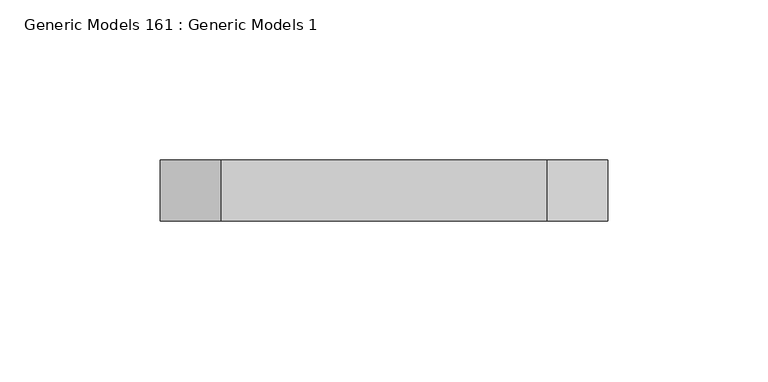
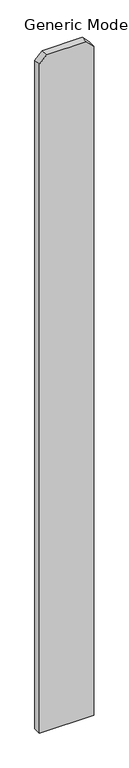
"""IFC4 building model written with IfcOpenShell, lengths in millimetres: proxy geometry, Generic Models 161 : Generic Models 1."""

import ifcopenshell
import ifcopenshell.guid

model = None  # the IFC model being written
_history = None  # IfcOwnerHistory: only IFC2X3 demands one
_inside = {}  # id of a spatial element -> (the spatial element, [elements in it])
_under = {}  # id of a project, library or spatial element -> (it, [spatial elements below it])
_declared = {}  # id of a project -> (the project, [libraries it declares])
_typed = {}  # id of a type object -> (the type object, [elements of that type])
_made_of = {}  # id of a material, layer set ... -> (it, [elements and type objects made of it])


def new_model(schema):
    """Start an empty IFC model of exactly this schema.

    Asked for "IFC4X3", IfcOpenShell would pick the latest addendum, in which some entities
    have other attributes; the version numbers below select the first issue.
    IFC2X3 requires an IfcOwnerHistory on every rooted entity: one is made here for all.
    """
    global model, _history
    if schema == "IFC4X3":
        model = ifcopenshell.file(schema_version=(4, 3, 0, 0))
    else:
        model = ifcopenshell.file(schema=schema)
    _inside.clear()
    _under.clear()
    _declared.clear()
    _typed.clear()
    _made_of.clear()
    _history = None
    if model.schema == "IFC2X3":
        org = make("IfcOrganization", Name="unknown")
        user = make(
            "IfcPersonAndOrganization",
            ThePerson=make("IfcPerson", FamilyName="unknown"),
            TheOrganization=org,
        )
        app = make(
            "IfcApplication",
            ApplicationDeveloper=org,
            Version="unknown",
            ApplicationFullName="unknown",
            ApplicationIdentifier="unknown",
        )
        _history = make(
            "IfcOwnerHistory",
            OwningUser=user,
            OwningApplication=app,
            ChangeAction="ADDED",
            CreationDate=0,
        )
    return model


def make(cls, **values):
    """One entity of the class cls with the attributes given. An attribute that is None is left unset."""
    return model.create_entity(
        cls, **{name: value for name, value in values.items() if value is not None}
    )


def rooted(cls, **values):
    """An entity with a GlobalId (a new one), such as an element, a storey or a relation."""
    return make(cls, GlobalId=ifcopenshell.guid.new(), OwnerHistory=_history, **values)


def si_unit(unit_type, name, prefix=None):
    """IfcSIUnit, for example si_unit("LENGTHUNIT", "METRE", prefix="MILLI")."""
    return make("IfcSIUnit", UnitType=unit_type, Prefix=prefix, Name=name)


def assignment(units):
    """IfcUnitAssignment: the units of a project."""
    return None if units is None else make("IfcUnitAssignment", Units=units)


def point(xyz):
    """IfcCartesianPoint."""
    return None if xyz is None else make("IfcCartesianPoint", Coordinates=xyz)


def direction(xyz):
    """IfcDirection."""
    return None if xyz is None else make("IfcDirection", DirectionRatios=xyz)


def frame(location, z_axis=None, x_axis=None):
    """IfcAxis2Placement3D, a coordinate frame: its origin and axes. An axis left out is left unset."""
    return make(
        "IfcAxis2Placement3D",
        Location=point(location),
        Axis=direction(z_axis),
        RefDirection=direction(x_axis),
    )


def origin():
    """The frame at (0, 0, 0) with its axes left unset."""
    return frame((0.0, 0.0, 0.0))


def place(relative_to, where):
    """IfcLocalPlacement: puts the frame where relative to a parent placement (None: the world)."""
    return make(
        "IfcLocalPlacement", PlacementRelTo=relative_to, RelativePlacement=where
    )


def context(
    kind, dimensions, precision=None, world=None, true_north=None, identifier=None
):
    """IfcGeometricRepresentationContext, for example the 3D "Model" context."""
    return make(
        "IfcGeometricRepresentationContext",
        ContextIdentifier=identifier,
        ContextType=kind,
        CoordinateSpaceDimension=dimensions,
        Precision=precision,
        WorldCoordinateSystem=world,
        TrueNorth=true_north,
    )


def project(units=None, contexts=None):
    """IfcProject with its units and contexts."""
    return rooted(
        "IfcProject",
        Name="project",
        RepresentationContexts=contexts,
        UnitsInContext=assignment(units),
    )


def spatial(cls, under=None, at=None, **own):
    """A site, building, storey or space (cls), placed at a placement, below another one or the project."""
    s = rooted(cls, ObjectPlacement=at, **own)
    if under is not None:
        _under.setdefault(under.id(), (under, []))[1].append(s)
    return s


def polyline(points):
    """IfcPolyline through the points."""
    return make("IfcPolyline", Points=[point(p) for p in points])


def outline(outer, holes=None, kind="AREA"):
    """IfcArbitraryClosedProfileDef: a profile drawn as a closed curve; with holes, ...WithVoids."""
    if holes is None:
        return make("IfcArbitraryClosedProfileDef", ProfileType=kind, OuterCurve=outer)
    return make(
        "IfcArbitraryProfileDefWithVoids",
        ProfileType=kind,
        OuterCurve=outer,
        InnerCurves=holes,
    )


def extrude(swept, where, along, depth):
    """IfcExtrudedAreaSolid: the profile swept, set in the frame where, extruded along a direction by depth."""
    return make(
        "IfcExtrudedAreaSolid",
        SweptArea=swept,
        Position=where,
        ExtrudedDirection=direction(along),
        Depth=depth,
    )


def shape(context_of_items, identifier, shape_type, items):
    """IfcShapeRepresentation: the items that make up one representation, for example the "Body"."""
    return make(
        "IfcShapeRepresentation",
        ContextOfItems=context_of_items,
        RepresentationIdentifier=identifier,
        RepresentationType=shape_type,
        Items=items,
    )


def source(mapping_origin, context_of_items, identifier, shape_type, items):
    """IfcRepresentationMap: a shape defined once, which mapped items show again and again."""
    return make(
        "IfcRepresentationMap",
        MappingOrigin=mapping_origin,
        MappedRepresentation=shape(context_of_items, identifier, shape_type, items),
    )


def transform(
    local_origin,
    x_axis=None,
    y_axis=None,
    z_axis=None,
    scale=None,
    scale2=None,
    scale3=None,
    uniform=True,
):
    """IfcCartesianTransformationOperator3D, or its non-uniform kind. x_axis, y_axis, z_axis: its Axis1, 2, 3."""
    if uniform:
        return make(
            "IfcCartesianTransformationOperator3D",
            Axis1=direction(x_axis),
            Axis2=direction(y_axis),
            LocalOrigin=point(local_origin),
            Scale=scale,
            Axis3=direction(z_axis),
        )
    return make(
        "IfcCartesianTransformationOperator3DnonUniform",
        Axis1=direction(x_axis),
        Axis2=direction(y_axis),
        LocalOrigin=point(local_origin),
        Scale=scale,
        Axis3=direction(z_axis),
        Scale2=scale2,
        Scale3=scale3,
    )


def mapped(mapping_source, mapping_target):
    """IfcMappedItem: shows the shape of a source again, moved by a transform."""
    return make(
        "IfcMappedItem", MappingSource=mapping_source, MappingTarget=mapping_target
    )


def made_of(thing, what):
    """Note that an element or type object is made of a material, layer set ...; save() writes the relation."""
    if what is not None:
        _made_of.setdefault(what.id(), (what, []))[1].append(thing)
    return thing


def element(
    cls,
    number,
    at=None,
    inside=None,
    cuts=None,
    type_object=None,
    material=None,
    context=None,
    identifier="Body",
    shape_type=None,
    held_by="IfcProductDefinitionShape",
    body=None,
    shapes=None,
    **own,
):
    """One element of the class cls, such as IfcWall. Its Tag is "e" and its number.

    at: its placement. inside: the storey or other place that contains it. cuts: it is an
    opening in that element (IfcRelVoidsElement). A single representation is given by context,
    identifier, shape_type and body (its items); several are given by shapes. held_by: the class
    of the entity that holds the representations. save() writes the other relations.
    """
    e = rooted(cls, Tag="e%d" % number, ObjectPlacement=at, **own)
    if body is not None:
        shapes = [shape(context, identifier, shape_type, body)]
    if shapes is not None:
        e.Representation = make(held_by, Representations=shapes)
    if inside is not None:
        _inside.setdefault(inside.id(), (inside, []))[1].append(e)
    if cuts is not None:
        rooted(
            "IfcRelVoidsElement", RelatingBuildingElement=cuts, RelatedOpeningElement=e
        )
    if type_object is not None:
        _typed.setdefault(type_object.id(), (type_object, []))[1].append(e)
    return made_of(e, material)


def aggregate(whole, parts):
    """IfcRelAggregates: a whole, such as a stair, and the parts it consists of."""
    return rooted("IfcRelAggregates", RelatingObject=whole, RelatedObjects=parts)


def save(model, path):
    """Write the relations noted so far, then the file.

    IfcRelAggregates (storeys below a building ...), IfcRelContainedInSpatialStructure (elements
    in a storey), IfcRelDefinesByType, IfcRelAssociatesMaterial and IfcRelDeclares: one each for
    every whole, place, type object, material and project.
    """
    for whole, parts in _under.values():
        aggregate(whole, parts)
    for where, things in _inside.values():
        rooted(
            "IfcRelContainedInSpatialStructure",
            RelatedElements=things,
            RelatingStructure=where,
        )
    for kind, things in _typed.values():
        rooted("IfcRelDefinesByType", RelatedObjects=things, RelatingType=kind)
    for what, things in _made_of.values():
        rooted("IfcRelAssociatesMaterial", RelatedObjects=things, RelatingMaterial=what)
    for by, libraries in _declared.values():
        rooted("IfcRelDeclares", RelatingContext=by, RelatedDefinitions=libraries)
    model.write(path)


def generic_models_161_generic_models_1_fa77210a(model_context):
    return source(origin(), model_context, "Body", "SweptSolid", [
        extrude(outline(polyline([(76.2, 54532.2125), (1885.95, 54532.2125), (1905.0, 54513.1625), (1905.0, 54411.5625), (1885.95, 54392.5125), (76.2, 54392.5125), (76.2, 54532.2125)])), frame((0.0, 547.6875, 0.0), z_axis=(0.0, 1.0, 0.0), x_axis=(0.0, 0.0, 1.0)), (0.0, 0.0, 1.0), 19.05),
    ])


if __name__ == "__main__":
    model = new_model("IFC4")
    model_context = context("Model", 3, world=origin())
    ifc_project = project(units=[si_unit("LENGTHUNIT", "METRE", prefix="MILLI")], contexts=[model_context])
    site = spatial("IfcSite", under=ifc_project)
    building = spatial("IfcBuilding", under=site)
    placement = place(None, origin())
    generic_models_161_generic_models_1_shape = generic_models_161_generic_models_1_fa77210a(model_context)
    element("IfcBuildingElementProxy", 1, Name="Generic Models 161 : Generic Models 1", ObjectType="Generic Models 161 : Generic Models 1", at=placement, inside=building, context=model_context, shape_type="MappedRepresentation", body=[
        mapped(generic_models_161_generic_models_1_shape, transform((0.0, 0.0, 0.0), x_axis=(1.0, 0.0, 0.0), y_axis=(0.0, 1.0, 0.0), z_axis=(0.0, 0.0, 1.0))),
    ])
    save(model, "model.ifc")

# Revit data of these elements
# Element 1 (IfcBuildingElementProxy, "Generic Models 161 : Generic Models 1")
#   Materials on its faces: "VERTICAL 1X6 CEDAR PLANKS W/ CLEAR WOOD SEALER"
# Materials
#   "VERTICAL 1X6 CEDAR PLANKS W/ CLEAR WOOD SEALER": class "Wood", colour RGB 234 198 147, transparency 0, Description = "Pinus Echinata", Cost = 0
